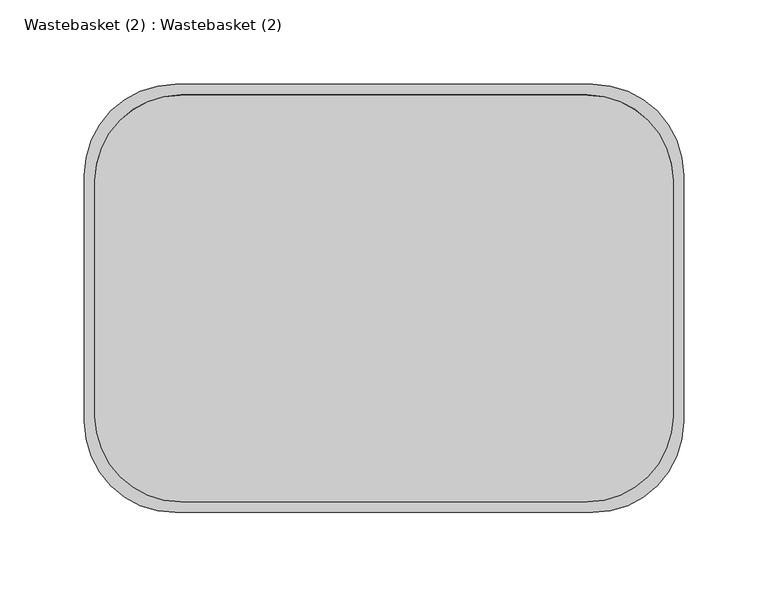
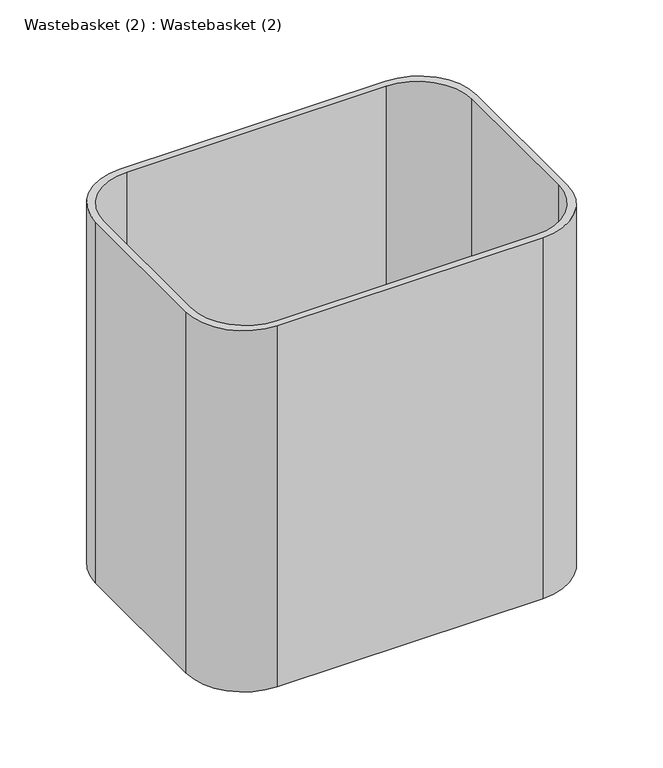
"""IFC4 building model written with IfcOpenShell, lengths in millimetres: furniture geometry, Wastebasket (2) : Wastebasket (2)."""

import ifcopenshell
import ifcopenshell.guid

model = None  # the IFC model being written
_history = None  # IfcOwnerHistory: only IFC2X3 demands one
_inside = {}  # id of a spatial element -> (the spatial element, [elements in it])
_under = {}  # id of a project, library or spatial element -> (it, [spatial elements below it])
_declared = {}  # id of a project -> (the project, [libraries it declares])
_typed = {}  # id of a type object -> (the type object, [elements of that type])
_made_of = {}  # id of a material, layer set ... -> (it, [elements and type objects made of it])


def new_model(schema):
    """Start an empty IFC model of exactly this schema.

    Asked for "IFC4X3", IfcOpenShell would pick the latest addendum, in which some entities
    have other attributes; the version numbers below select the first issue.
    IFC2X3 requires an IfcOwnerHistory on every rooted entity: one is made here for all.
    """
    global model, _history
    if schema == "IFC4X3":
        model = ifcopenshell.file(schema_version=(4, 3, 0, 0))
    else:
        model = ifcopenshell.file(schema=schema)
    _inside.clear()
    _under.clear()
    _declared.clear()
    _typed.clear()
    _made_of.clear()
    _history = None
    if model.schema == "IFC2X3":
        org = make("IfcOrganization", Name="unknown")
        user = make(
            "IfcPersonAndOrganization",
            ThePerson=make("IfcPerson", FamilyName="unknown"),
            TheOrganization=org,
        )
        app = make(
            "IfcApplication",
            ApplicationDeveloper=org,
            Version="unknown",
            ApplicationFullName="unknown",
            ApplicationIdentifier="unknown",
        )
        _history = make(
            "IfcOwnerHistory",
            OwningUser=user,
            OwningApplication=app,
            ChangeAction="ADDED",
            CreationDate=0,
        )
    return model


def make(cls, **values):
    """One entity of the class cls with the attributes given. An attribute that is None is left unset."""
    return model.create_entity(
        cls, **{name: value for name, value in values.items() if value is not None}
    )


def rooted(cls, **values):
    """An entity with a GlobalId (a new one), such as an element, a storey or a relation."""
    return make(cls, GlobalId=ifcopenshell.guid.new(), OwnerHistory=_history, **values)


def si_unit(unit_type, name, prefix=None):
    """IfcSIUnit, for example si_unit("LENGTHUNIT", "METRE", prefix="MILLI")."""
    return make("IfcSIUnit", UnitType=unit_type, Prefix=prefix, Name=name)


def assignment(units):
    """IfcUnitAssignment: the units of a project."""
    return None if units is None else make("IfcUnitAssignment", Units=units)


def point(xyz):
    """IfcCartesianPoint."""
    return None if xyz is None else make("IfcCartesianPoint", Coordinates=xyz)


def direction(xyz):
    """IfcDirection."""
    return None if xyz is None else make("IfcDirection", DirectionRatios=xyz)


def frame(location, z_axis=None, x_axis=None):
    """IfcAxis2Placement3D, a coordinate frame: its origin and axes. An axis left out is left unset."""
    return make(
        "IfcAxis2Placement3D",
        Location=point(location),
        Axis=direction(z_axis),
        RefDirection=direction(x_axis),
    )


def origin():
    """The frame at (0, 0, 0) with its axes left unset."""
    return frame((0.0, 0.0, 0.0))


def place(relative_to, where):
    """IfcLocalPlacement: puts the frame where relative to a parent placement (None: the world)."""
    return make(
        "IfcLocalPlacement", PlacementRelTo=relative_to, RelativePlacement=where
    )


def context(
    kind, dimensions, precision=None, world=None, true_north=None, identifier=None
):
    """IfcGeometricRepresentationContext, for example the 3D "Model" context."""
    return make(
        "IfcGeometricRepresentationContext",
        ContextIdentifier=identifier,
        ContextType=kind,
        CoordinateSpaceDimension=dimensions,
        Precision=precision,
        WorldCoordinateSystem=world,
        TrueNorth=true_north,
    )


def project(units=None, contexts=None):
    """IfcProject with its units and contexts."""
    return rooted(
        "IfcProject",
        Name="project",
        RepresentationContexts=contexts,
        UnitsInContext=assignment(units),
    )


def spatial(cls, under=None, at=None, **own):
    """A site, building, storey or space (cls), placed at a placement, below another one or the project."""
    s = rooted(cls, ObjectPlacement=at, **own)
    if under is not None:
        _under.setdefault(under.id(), (under, []))[1].append(s)
    return s


def polyline(points):
    """IfcPolyline through the points."""
    return make("IfcPolyline", Points=[point(p) for p in points])


def circle_curve(where, radius):
    """IfcCircle in the frame where."""
    return make("IfcCircle", Position=where, Radius=radius)


def shape(context_of_items, identifier, shape_type, items):
    """IfcShapeRepresentation: the items that make up one representation, for example the "Body"."""
    return make(
        "IfcShapeRepresentation",
        ContextOfItems=context_of_items,
        RepresentationIdentifier=identifier,
        RepresentationType=shape_type,
        Items=items,
    )


def source(mapping_origin, context_of_items, identifier, shape_type, items):
    """IfcRepresentationMap: a shape defined once, which mapped items show again and again."""
    return make(
        "IfcRepresentationMap",
        MappingOrigin=mapping_origin,
        MappedRepresentation=shape(context_of_items, identifier, shape_type, items),
    )


def transform(
    local_origin,
    x_axis=None,
    y_axis=None,
    z_axis=None,
    scale=None,
    scale2=None,
    scale3=None,
    uniform=True,
):
    """IfcCartesianTransformationOperator3D, or its non-uniform kind. x_axis, y_axis, z_axis: its Axis1, 2, 3."""
    if uniform:
        return make(
            "IfcCartesianTransformationOperator3D",
            Axis1=direction(x_axis),
            Axis2=direction(y_axis),
            LocalOrigin=point(local_origin),
            Scale=scale,
            Axis3=direction(z_axis),
        )
    return make(
        "IfcCartesianTransformationOperator3DnonUniform",
        Axis1=direction(x_axis),
        Axis2=direction(y_axis),
        LocalOrigin=point(local_origin),
        Scale=scale,
        Axis3=direction(z_axis),
        Scale2=scale2,
        Scale3=scale3,
    )


def mapped(mapping_source, mapping_target):
    """IfcMappedItem: shows the shape of a source again, moved by a transform."""
    return make(
        "IfcMappedItem", MappingSource=mapping_source, MappingTarget=mapping_target
    )


def made_of(thing, what):
    """Note that an element or type object is made of a material, layer set ...; save() writes the relation."""
    if what is not None:
        _made_of.setdefault(what.id(), (what, []))[1].append(thing)
    return thing


def element(
    cls,
    number,
    at=None,
    inside=None,
    cuts=None,
    type_object=None,
    material=None,
    context=None,
    identifier="Body",
    shape_type=None,
    held_by="IfcProductDefinitionShape",
    body=None,
    shapes=None,
    **own,
):
    """One element of the class cls, such as IfcWall. Its Tag is "e" and its number.

    at: its placement. inside: the storey or other place that contains it. cuts: it is an
    opening in that element (IfcRelVoidsElement). A single representation is given by context,
    identifier, shape_type and body (its items); several are given by shapes. held_by: the class
    of the entity that holds the representations. save() writes the other relations.
    """
    e = rooted(cls, Tag="e%d" % number, ObjectPlacement=at, **own)
    if body is not None:
        shapes = [shape(context, identifier, shape_type, body)]
    if shapes is not None:
        e.Representation = make(held_by, Representations=shapes)
    if inside is not None:
        _inside.setdefault(inside.id(), (inside, []))[1].append(e)
    if cuts is not None:
        rooted(
            "IfcRelVoidsElement", RelatingBuildingElement=cuts, RelatedOpeningElement=e
        )
    if type_object is not None:
        _typed.setdefault(type_object.id(), (type_object, []))[1].append(e)
    return made_of(e, material)


def aggregate(whole, parts):
    """IfcRelAggregates: a whole, such as a stair, and the parts it consists of."""
    return rooted("IfcRelAggregates", RelatingObject=whole, RelatedObjects=parts)


def save(model, path):
    """Write the relations noted so far, then the file.

    IfcRelAggregates (storeys below a building ...), IfcRelContainedInSpatialStructure (elements
    in a storey), IfcRelDefinesByType, IfcRelAssociatesMaterial and IfcRelDeclares: one each for
    every whole, place, type object, material and project.
    """
    for whole, parts in _under.values():
        aggregate(whole, parts)
    for where, things in _inside.values():
        rooted(
            "IfcRelContainedInSpatialStructure",
            RelatedElements=things,
            RelatingStructure=where,
        )
    for kind, things in _typed.values():
        rooted("IfcRelDefinesByType", RelatedObjects=things, RelatingType=kind)
    for what, things in _made_of.values():
        rooted("IfcRelAssociatesMaterial", RelatedObjects=things, RelatingMaterial=what)
    for by, libraries in _declared.values():
        rooted("IfcRelDeclares", RelatingContext=by, RelatedDefinitions=libraries)
    model.write(path)


def plane_surface(at):
    """IfcPlane: the flat surface through the origin of the frame at, square to its z axis."""
    return make("IfcPlane", Position=at)


def cylinder_surface(at, radius):
    """IfcCylindricalSurface: all points at the distance radius from the z axis of the frame at."""
    return make("IfcCylindricalSurface", Position=at, Radius=radius)


def revolved_surface(curve, axis_point, axis_direction):
    """IfcSurfaceOfRevolution: the curve turned about the line through axis_point along axis_direction."""
    return make(
        "IfcSurfaceOfRevolution",
        SweptCurve=make("IfcArbitraryOpenProfileDef", ProfileType="CURVE", Curve=curve),
        AxisPosition=make("IfcAxis1Placement", Location=point(axis_point), Axis=direction(axis_direction)),
    )


def advanced_brep(points, edges, surfaces, faces):
    """IfcAdvancedBrep: a solid bounded by faces that lie on surfaces and meet in shared edges.

    An edge is (start, end): straight between two places in points (the first is 0);
    or (start, end, curve); or (start, end, curve, False) where it runs against its curve.
    A face is (place in surfaces, loops), or (place, loops, False) where it looks against
    its surface's normal. A loop lists edges by number (the first is 1), with a minus sign
    where the edge is run from its end to its start. The first loop is the outer one.
    """
    corners = [point(p) for p in points]
    vertices = [make("IfcVertexPoint", VertexGeometry=c) for c in corners]
    made = []
    for start, end, *more in edges:
        made.append(
            make(
                "IfcEdgeCurve",
                EdgeStart=vertices[start],
                EdgeEnd=vertices[end],
                EdgeGeometry=more[0] if more else make("IfcPolyline", Points=[corners[start], corners[end]]),
                SameSense=more[1] if len(more) > 1 else True,
            )
        )
    hull = []
    for where, loops, *sense in faces:
        bounds = []
        for j, loop in enumerate(loops):
            ring = [make("IfcOrientedEdge", EdgeElement=made[abs(k) - 1], Orientation=k > 0) for k in loop]
            bounds.append(
                make(
                    "IfcFaceOuterBound" if j == 0 else "IfcFaceBound",
                    Bound=make("IfcEdgeLoop", EdgeList=ring),
                    Orientation=True,
                )
            )
        hull.append(make("IfcAdvancedFace", Bounds=bounds, FaceSurface=surfaces[where], SameSense=sense[0] if sense else True))
    return make("IfcAdvancedBrep", Outer=make("IfcClosedShell", CfsFaces=hull))


def wastebasket_2_wastebasket_2_e1224e57(model_context):
    return source(origin(), model_context, "Body", "AdvancedBrep", [
        advanced_brep(
        [(178.3203994, 170.9615385, 355.6), (-69.3296006, 170.9615385, 355.6), (-123.3046006, 116.9865385, 355.6), (-123.3046006, -29.0634615, 355.6), (-69.3296006, -83.0384615, 355.6), (178.3203994, -83.0384615, 355.6), (232.2953994, -29.0634615, 355.6), (232.2953994, 116.9865385, 355.6), (-66.1546006, 164.6115385, 355.6), (175.1453994, 164.6115385, 355.6), (225.9453994, 113.8115385, 355.6), (225.9453994, -25.8884615, 355.6), (175.1453994, -76.6884615, 355.6), (-66.1546006, -76.6884615, 355.6), (-116.9546006, -25.8884615, 355.6), (-116.9546006, 113.8115385, 355.6), (178.3203994, 170.9615385, 0.0), (232.2953994, 116.9865385, 0.0), (232.2953994, -29.0634615, 0.0), (178.3203994, -83.0384615, 0.0), (-69.3296006, -83.0384615, 0.0), (-123.3046006, -29.0634615, 0.0), (-123.3046006, 116.9865385, 0.0), (-69.3296006, 170.9615385, 0.0), (175.1453994, 164.6115385, 12.7), (-66.1546006, 164.6115385, 12.7), (-116.9546006, 113.8115385, 12.7), (-116.9546006, -25.8884615, 12.7), (-66.1546006, -76.6884615, 12.7), (175.1453994, -76.6884615, 12.7), (225.9453994, -25.8884615, 12.7), (225.9453994, 113.8115385, 12.7)],
        [
            (0, 1),
            (1, 2, circle_curve(frame((-69.3296006, 116.9865385, 355.6), z_axis=(0.0, 0.0, 1.0), x_axis=(1.0, 0.0, 0.0)), 53.975)),
            (2, 3),
            (3, 4, circle_curve(frame((-69.3296006, -29.0634615, 355.6), z_axis=(0.0, 0.0, 1.0), x_axis=(1.0, 0.0, 0.0)), 53.975)),
            (4, 5),
            (5, 6, circle_curve(frame((178.3203994, -29.0634615, 355.6), z_axis=(0.0, 0.0, 1.0), x_axis=(1.0, 0.0, 0.0)), 53.975)),
            (6, 7),
            (7, 0, circle_curve(frame((178.3203994, 116.9865385, 355.6), z_axis=(0.0, 0.0, 1.0), x_axis=(1.0, 0.0, 0.0)), 53.975)),
            (8, 9),
            (9, 10, circle_curve(frame((175.1453994, 113.8115385, 355.6), z_axis=(0.0, 0.0, -1.0), x_axis=(1.0, 0.0, 0.0)), 50.8)),
            (10, 11),
            (11, 12, circle_curve(frame((175.1453994, -25.8884615, 355.6), z_axis=(0.0, 0.0, -1.0), x_axis=(1.0, 0.0, 0.0)), 50.8)),
            (12, 13),
            (13, 14, circle_curve(frame((-66.1546006, -25.8884615, 355.6), z_axis=(0.0, 0.0, -1.0), x_axis=(1.0, 0.0, 0.0)), 50.8)),
            (14, 15),
            (15, 8, circle_curve(frame((-66.1546006, 113.8115385, 355.6), z_axis=(0.0, 0.0, -1.0), x_axis=(1.0, 0.0, 0.0)), 50.8)),
            (16, 17, circle_curve(frame((178.3203994, 116.9865385, 0.0), z_axis=(0.0, 0.0, -1.0), x_axis=(1.0, 0.0, 0.0)), 53.975)),
            (17, 18),
            (18, 19, circle_curve(frame((178.3203994, -29.0634615, 0.0), z_axis=(0.0, 0.0, -1.0), x_axis=(1.0, 0.0, 0.0)), 53.975)),
            (19, 20),
            (20, 21, circle_curve(frame((-69.3296006, -29.0634615, 0.0), z_axis=(0.0, 0.0, -1.0), x_axis=(1.0, 0.0, 0.0)), 53.975)),
            (21, 22),
            (22, 23, circle_curve(frame((-69.3296006, 116.9865385, 0.0), z_axis=(0.0, 0.0, -1.0), x_axis=(1.0, 0.0, 0.0)), 53.975)),
            (23, 16),
            (0, 16),
            (23, 1),
            (22, 2),
            (21, 3),
            (20, 4),
            (19, 5),
            (18, 6),
            (17, 7),
            (24, 25),
            (25, 26, circle_curve(frame((-66.1546006, 113.8115385, 12.7), z_axis=(0.0, 0.0, 1.0), x_axis=(1.0, 0.0, 0.0)), 50.8)),
            (26, 27),
            (27, 28, circle_curve(frame((-66.1546006, -25.8884615, 12.7), z_axis=(0.0, 0.0, 1.0), x_axis=(1.0, 0.0, 0.0)), 50.8)),
            (28, 29),
            (29, 30, circle_curve(frame((175.1453994, -25.8884615, 12.7), z_axis=(0.0, 0.0, 1.0), x_axis=(1.0, 0.0, 0.0)), 50.8)),
            (30, 31),
            (31, 24, circle_curve(frame((175.1453994, 113.8115385, 12.7), z_axis=(0.0, 0.0, 1.0), x_axis=(1.0, 0.0, 0.0)), 50.8)),
            (24, 9),
            (8, 25),
            (15, 26),
            (14, 27),
            (13, 28),
            (12, 29),
            (11, 30),
            (10, 31),
        ],
        [
            plane_surface(frame((-123.3046006, 170.9615385, 355.6), z_axis=(0.0, 0.0, 1.0), x_axis=(-1.0, 0.0, 0.0))),
            plane_surface(frame((-123.3046006, 170.9615385, 0.0), z_axis=(0.0, 0.0, -1.0), x_axis=(1.0, 0.0, 0.0))),
            plane_surface(frame((178.3203994, 170.9615385, 355.6), z_axis=(0.0, 1.0, 0.0), x_axis=(0.0, 0.0, -1.0))),
            cylinder_surface(frame((-69.3296006, 116.9865385, 0.0), z_axis=(0.0, 0.0, 1.0), x_axis=(1.0, 0.0, 0.0)), 53.975),
            plane_surface(frame((-123.3046006, 116.9865385, 355.6), z_axis=(-1.0, 0.0, 0.0), x_axis=(0.0, 0.0, -1.0))),
            cylinder_surface(frame((-69.3296006, -29.0634615, 0.0), z_axis=(0.0, 0.0, 1.0), x_axis=(1.0, 0.0, 0.0)), 53.975),
            plane_surface(frame((-69.3296006, -83.0384615, 355.6), z_axis=(0.0, -1.0, 0.0), x_axis=(0.0, 0.0, -1.0))),
            cylinder_surface(frame((178.3203994, -29.0634615, 0.0), z_axis=(0.0, 0.0, 1.0), x_axis=(1.0, 0.0, 0.0)), 53.975),
            plane_surface(frame((232.2953994, -29.0634615, 355.6), z_axis=(1.0, 0.0, 0.0), x_axis=(0.0, 0.0, -1.0))),
            cylinder_surface(frame((178.3203994, 116.9865385, 0.0), z_axis=(0.0, 0.0, 1.0), x_axis=(1.0, 0.0, 0.0)), 53.975),
            plane_surface(frame((-66.1546006, 164.6115385, 12.7), z_axis=(0.0, 0.0, 1.0), x_axis=(1.0, 0.0, 0.0))),
            plane_surface(frame((175.1453994, 164.6115385, 355.6), z_axis=(0.0, -1.0, 0.0), x_axis=(0.0, 0.0, -1.0))),
            revolved_surface(polyline([(-15.354600599999998, 113.8115385, 355.6), (-15.354600599999998, 113.8115385, 12.7)]), (-66.1546006, 113.8115385, 12.7), (0.0, 0.0, 1.0)),
            plane_surface(frame((-116.9546006, 113.8115385, 355.6), z_axis=(1.0, 0.0, 0.0), x_axis=(0.0, 0.0, -1.0))),
            revolved_surface(polyline([(-15.354600599999998, -25.8884615, 355.6), (-15.354600599999998, -25.8884615, 12.7)]), (-66.1546006, -25.8884615, 12.7), (0.0, 0.0, 1.0)),
            plane_surface(frame((-66.1546006, -76.6884615, 355.6), z_axis=(0.0, 1.0, 0.0), x_axis=(0.0, 0.0, -1.0))),
            revolved_surface(polyline([(225.94539939999999, -25.8884615, 355.6), (225.94539939999999, -25.8884615, 12.7)]), (175.1453994, -25.8884615, 12.7), (0.0, 0.0, 1.0)),
            plane_surface(frame((225.9453994, -25.8884615, 355.6), z_axis=(-1.0, 0.0, 0.0), x_axis=(0.0, 0.0, -1.0))),
            revolved_surface(polyline([(225.94539939999999, 113.8115385, 355.6), (225.94539939999999, 113.8115385, 12.7)]), (175.1453994, 113.8115385, 12.7), (0.0, 0.0, 1.0)),
        ],
        [
            (0, [[1, 2, 3, 4, 5, 6, 7, 8], [9, 10, 11, 12, 13, 14, 15, 16]]),
            (1, [[17, 18, 19, 20, 21, 22, 23, 24]]),
            (2, [[-1, 25, -24, 26]]),
            (3, [[-2, -26, -23, 27]]),
            (4, [[-3, -27, -22, 28]]),
            (5, [[-4, -28, -21, 29]]),
            (6, [[-5, -29, -20, 30]]),
            (7, [[-6, -30, -19, 31]]),
            (8, [[-7, -31, -18, 32]]),
            (9, [[-8, -32, -17, -25]]),
            (10, [[33, 34, 35, 36, 37, 38, 39, 40]]),
            (11, [[-33, 41, -9, 42]]),
            (12, [[-34, -42, -16, 43]]),
            (13, [[-35, -43, -15, 44]]),
            (14, [[-36, -44, -14, 45]]),
            (15, [[-37, -45, -13, 46]]),
            (16, [[-38, -46, -12, 47]]),
            (17, [[-39, -47, -11, 48]]),
            (18, [[-40, -48, -10, -41]]),
        ],
    ),
    ])


if __name__ == "__main__":
    model = new_model("IFC4")
    model_context = context("Model", 3, world=origin())
    ifc_project = project(units=[si_unit("LENGTHUNIT", "METRE", prefix="MILLI")], contexts=[model_context])
    site = spatial("IfcSite", under=ifc_project)
    building = spatial("IfcBuilding", under=site)
    placement = place(None, origin())
    wastebasket_2_wastebasket_2_shape = wastebasket_2_wastebasket_2_e1224e57(model_context)
    element("IfcFurniture", 1, ObjectType="Wastebasket (2) : Wastebasket (2)", at=placement, inside=building, context=model_context, shape_type="MappedRepresentation", body=[
        mapped(wastebasket_2_wastebasket_2_shape, transform((0.0, 0.0, 0.0), x_axis=(1.0, 0.0, 0.0), y_axis=(0.0, 1.0, 0.0), z_axis=(0.0, 0.0, 1.0))),
    ])
    save(model, "model.ifc")

# Revit data of these elements
# Type "Wastebasket (2) : Wastebasket (2)"
#   Keynote = "N"
#   Material Bin = Metal - Chrome
#   Default Elevation = 0
#   Assembly Code = ""
# Element 1 (IfcFurniture, "Wastebasket (2) : Wastebasket (2)")
#   Materials on its faces: "Metal - Chrome"
# Materials
#   "Metal - Chrome": class "Metal", colour RGB 206 206 206, transparency 0
